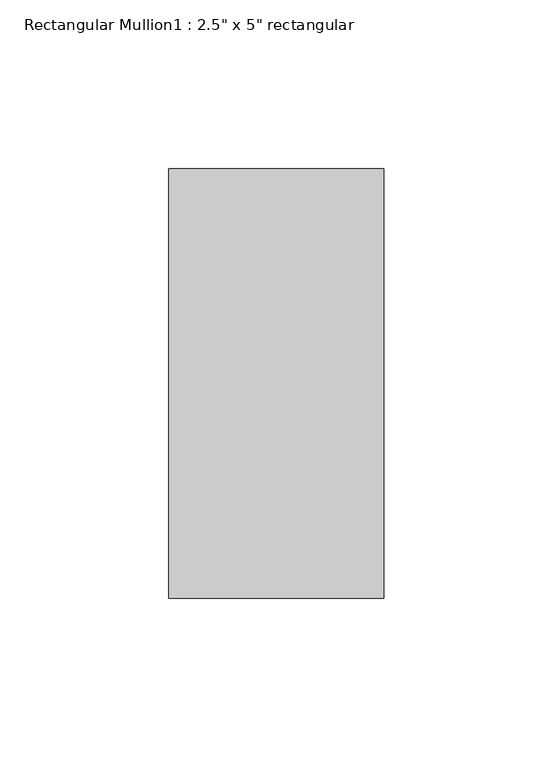
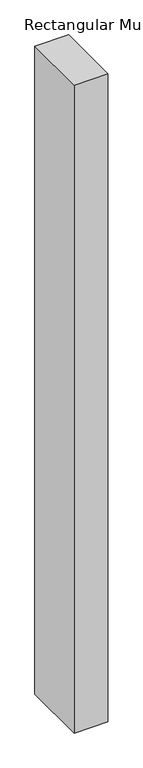
"""IFC4 building model written with IfcOpenShell, lengths in millimetres: member geometry."""

from ifc_helpers import new_model, si_unit, frame, origin, place, context, project, spatial, polyline, outline, extrude, source, transform, mapped, element, save


def member_5783932f(model_context):
    return source(origin(), model_context, "Body", "SweptSolid", [
        extrude(outline(polyline([(0.0, 63.5), (0.0, -63.5), (-63.5, -63.5), (-63.5, 63.5), (0.0, 63.5)])), frame((0.0, 0.0, -1282.7), z_axis=(0.0, 0.0, 1.0), x_axis=(1.0, 0.0, 0.0)), (0.0, 0.0, 1.0), 1282.7),
    ])


if __name__ == "__main__":
    model = new_model("IFC4")
    model_context = context("Model", 3, world=origin())
    ifc_project = project(units=[si_unit("LENGTHUNIT", "METRE", prefix="MILLI")], contexts=[model_context])
    site = spatial("IfcSite", under=ifc_project)
    building = spatial("IfcBuilding", under=site)
    placement = place(None, origin())
    member_shape = member_5783932f(model_context)
    element("IfcMember", 1, ObjectType="Rectangular Mullion1 : 2.5\" x 5\" rectangular", at=placement, inside=building, context=model_context, shape_type="MappedRepresentation", body=[
        mapped(member_shape, transform((0.0, 0.0, 0.0), x_axis=(1.0, 0.0, 0.0), y_axis=(0.0, 1.0, 0.0), z_axis=(0.0, 0.0, 1.0))),
    ])
    save(model, "model.ifc")

# Revit data of these elements
# Type "Rectangular Mullion1 : 2.5\" x 5\" rectangular"
#   built-in parameter 1007304 = 0.416667 (stored number, unit not read)
#   built-in parameter 1007301 = 0.104167 (stored number, unit not read)
#   built-in parameter 1007300 = 0.104167 (stored number, unit not read)
# Element 1 (IfcMember, "Rectangular Mullion1 : 2.5\" x 5\" rectangular")
#   Materials on its faces: "support-frame"
# Materials
#   "support-frame": class "Unassigned", colour RGB 233 233 233, transparency 0, Cost = 0
